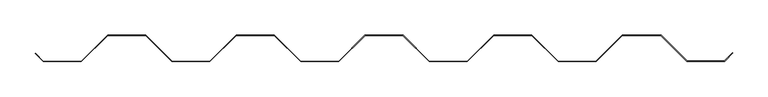
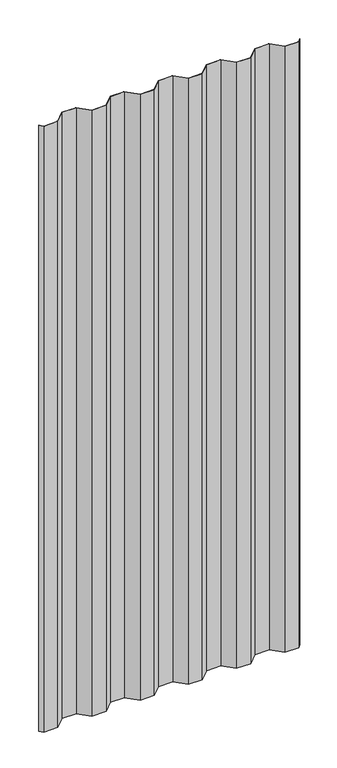
"""IFC4 building model written with IfcOpenShell, lengths in millimetres: proxy geometry, MBCI 7.2-V Panel-1 : MBCI 7.2-V Panel-1."""

import ifcopenshell
import ifcopenshell.guid

model = None  # the IFC model being written
_history = None  # IfcOwnerHistory: only IFC2X3 demands one
_inside = {}  # id of a spatial element -> (the spatial element, [elements in it])
_under = {}  # id of a project, library or spatial element -> (it, [spatial elements below it])
_declared = {}  # id of a project -> (the project, [libraries it declares])
_typed = {}  # id of a type object -> (the type object, [elements of that type])
_made_of = {}  # id of a material, layer set ... -> (it, [elements and type objects made of it])


def new_model(schema):
    """Start an empty IFC model of exactly this schema.

    Asked for "IFC4X3", IfcOpenShell would pick the latest addendum, in which some entities
    have other attributes; the version numbers below select the first issue.
    IFC2X3 requires an IfcOwnerHistory on every rooted entity: one is made here for all.
    """
    global model, _history
    if schema == "IFC4X3":
        model = ifcopenshell.file(schema_version=(4, 3, 0, 0))
    else:
        model = ifcopenshell.file(schema=schema)
    _inside.clear()
    _under.clear()
    _declared.clear()
    _typed.clear()
    _made_of.clear()
    _history = None
    if model.schema == "IFC2X3":
        org = make("IfcOrganization", Name="unknown")
        user = make(
            "IfcPersonAndOrganization",
            ThePerson=make("IfcPerson", FamilyName="unknown"),
            TheOrganization=org,
        )
        app = make(
            "IfcApplication",
            ApplicationDeveloper=org,
            Version="unknown",
            ApplicationFullName="unknown",
            ApplicationIdentifier="unknown",
        )
        _history = make(
            "IfcOwnerHistory",
            OwningUser=user,
            OwningApplication=app,
            ChangeAction="ADDED",
            CreationDate=0,
        )
    return model


def make(cls, **values):
    """One entity of the class cls with the attributes given. An attribute that is None is left unset."""
    return model.create_entity(
        cls, **{name: value for name, value in values.items() if value is not None}
    )


def rooted(cls, **values):
    """An entity with a GlobalId (a new one), such as an element, a storey or a relation."""
    return make(cls, GlobalId=ifcopenshell.guid.new(), OwnerHistory=_history, **values)


def si_unit(unit_type, name, prefix=None):
    """IfcSIUnit, for example si_unit("LENGTHUNIT", "METRE", prefix="MILLI")."""
    return make("IfcSIUnit", UnitType=unit_type, Prefix=prefix, Name=name)


def assignment(units):
    """IfcUnitAssignment: the units of a project."""
    return None if units is None else make("IfcUnitAssignment", Units=units)


def point(xyz):
    """IfcCartesianPoint."""
    return None if xyz is None else make("IfcCartesianPoint", Coordinates=xyz)


def direction(xyz):
    """IfcDirection."""
    return None if xyz is None else make("IfcDirection", DirectionRatios=xyz)


def frame(location, z_axis=None, x_axis=None):
    """IfcAxis2Placement3D, a coordinate frame: its origin and axes. An axis left out is left unset."""
    return make(
        "IfcAxis2Placement3D",
        Location=point(location),
        Axis=direction(z_axis),
        RefDirection=direction(x_axis),
    )


def origin():
    """The frame at (0, 0, 0) with its axes left unset."""
    return frame((0.0, 0.0, 0.0))


def place(relative_to, where):
    """IfcLocalPlacement: puts the frame where relative to a parent placement (None: the world)."""
    return make(
        "IfcLocalPlacement", PlacementRelTo=relative_to, RelativePlacement=where
    )


def context(
    kind, dimensions, precision=None, world=None, true_north=None, identifier=None
):
    """IfcGeometricRepresentationContext, for example the 3D "Model" context."""
    return make(
        "IfcGeometricRepresentationContext",
        ContextIdentifier=identifier,
        ContextType=kind,
        CoordinateSpaceDimension=dimensions,
        Precision=precision,
        WorldCoordinateSystem=world,
        TrueNorth=true_north,
    )


def project(units=None, contexts=None):
    """IfcProject with its units and contexts."""
    return rooted(
        "IfcProject",
        Name="project",
        RepresentationContexts=contexts,
        UnitsInContext=assignment(units),
    )


def spatial(cls, under=None, at=None, **own):
    """A site, building, storey or space (cls), placed at a placement, below another one or the project."""
    s = rooted(cls, ObjectPlacement=at, **own)
    if under is not None:
        _under.setdefault(under.id(), (under, []))[1].append(s)
    return s


def polyline(points):
    """IfcPolyline through the points."""
    return make("IfcPolyline", Points=[point(p) for p in points])


def outline(outer, holes=None, kind="AREA"):
    """IfcArbitraryClosedProfileDef: a profile drawn as a closed curve; with holes, ...WithVoids."""
    if holes is None:
        return make("IfcArbitraryClosedProfileDef", ProfileType=kind, OuterCurve=outer)
    return make(
        "IfcArbitraryProfileDefWithVoids",
        ProfileType=kind,
        OuterCurve=outer,
        InnerCurves=holes,
    )


def extrude(swept, where, along, depth):
    """IfcExtrudedAreaSolid: the profile swept, set in the frame where, extruded along a direction by depth."""
    return make(
        "IfcExtrudedAreaSolid",
        SweptArea=swept,
        Position=where,
        ExtrudedDirection=direction(along),
        Depth=depth,
    )


def shape(context_of_items, identifier, shape_type, items):
    """IfcShapeRepresentation: the items that make up one representation, for example the "Body"."""
    return make(
        "IfcShapeRepresentation",
        ContextOfItems=context_of_items,
        RepresentationIdentifier=identifier,
        RepresentationType=shape_type,
        Items=items,
    )


def source(mapping_origin, context_of_items, identifier, shape_type, items):
    """IfcRepresentationMap: a shape defined once, which mapped items show again and again."""
    return make(
        "IfcRepresentationMap",
        MappingOrigin=mapping_origin,
        MappedRepresentation=shape(context_of_items, identifier, shape_type, items),
    )


def transform(
    local_origin,
    x_axis=None,
    y_axis=None,
    z_axis=None,
    scale=None,
    scale2=None,
    scale3=None,
    uniform=True,
):
    """IfcCartesianTransformationOperator3D, or its non-uniform kind. x_axis, y_axis, z_axis: its Axis1, 2, 3."""
    if uniform:
        return make(
            "IfcCartesianTransformationOperator3D",
            Axis1=direction(x_axis),
            Axis2=direction(y_axis),
            LocalOrigin=point(local_origin),
            Scale=scale,
            Axis3=direction(z_axis),
        )
    return make(
        "IfcCartesianTransformationOperator3DnonUniform",
        Axis1=direction(x_axis),
        Axis2=direction(y_axis),
        LocalOrigin=point(local_origin),
        Scale=scale,
        Axis3=direction(z_axis),
        Scale2=scale2,
        Scale3=scale3,
    )


def mapped(mapping_source, mapping_target):
    """IfcMappedItem: shows the shape of a source again, moved by a transform."""
    return make(
        "IfcMappedItem", MappingSource=mapping_source, MappingTarget=mapping_target
    )


def made_of(thing, what):
    """Note that an element or type object is made of a material, layer set ...; save() writes the relation."""
    if what is not None:
        _made_of.setdefault(what.id(), (what, []))[1].append(thing)
    return thing


def element(
    cls,
    number,
    at=None,
    inside=None,
    cuts=None,
    type_object=None,
    material=None,
    context=None,
    identifier="Body",
    shape_type=None,
    held_by="IfcProductDefinitionShape",
    body=None,
    shapes=None,
    **own,
):
    """One element of the class cls, such as IfcWall. Its Tag is "e" and its number.

    at: its placement. inside: the storey or other place that contains it. cuts: it is an
    opening in that element (IfcRelVoidsElement). A single representation is given by context,
    identifier, shape_type and body (its items); several are given by shapes. held_by: the class
    of the entity that holds the representations. save() writes the other relations.
    """
    e = rooted(cls, Tag="e%d" % number, ObjectPlacement=at, **own)
    if body is not None:
        shapes = [shape(context, identifier, shape_type, body)]
    if shapes is not None:
        e.Representation = make(held_by, Representations=shapes)
    if inside is not None:
        _inside.setdefault(inside.id(), (inside, []))[1].append(e)
    if cuts is not None:
        rooted(
            "IfcRelVoidsElement", RelatingBuildingElement=cuts, RelatedOpeningElement=e
        )
    if type_object is not None:
        _typed.setdefault(type_object.id(), (type_object, []))[1].append(e)
    return made_of(e, material)


def aggregate(whole, parts):
    """IfcRelAggregates: a whole, such as a stair, and the parts it consists of."""
    return rooted("IfcRelAggregates", RelatingObject=whole, RelatedObjects=parts)


def save(model, path):
    """Write the relations noted so far, then the file.

    IfcRelAggregates (storeys below a building ...), IfcRelContainedInSpatialStructure (elements
    in a storey), IfcRelDefinesByType, IfcRelAssociatesMaterial and IfcRelDeclares: one each for
    every whole, place, type object, material and project.
    """
    for whole, parts in _under.values():
        aggregate(whole, parts)
    for where, things in _inside.values():
        rooted(
            "IfcRelContainedInSpatialStructure",
            RelatedElements=things,
            RelatingStructure=where,
        )
    for kind, things in _typed.values():
        rooted("IfcRelDefinesByType", RelatedObjects=things, RelatingType=kind)
    for what, things in _made_of.values():
        rooted("IfcRelAssociatesMaterial", RelatedObjects=things, RelatingMaterial=what)
    for by, libraries in _declared.values():
        rooted("IfcRelDeclares", RelatingContext=by, RelatedDefinitions=libraries)
    model.write(path)


def generic_models_de5cb4ec(model_context):
    return source(origin(), model_context, "Body", "SweptSolid", [
        extrude(outline(polyline([(589155.5303729, -531639.2163841), (589101.4186638, -531639.2163841), (589090.0180296, -531627.81575), (589090.8180038, -531627.7738251), (589101.6652503, -531638.6210716), (589155.2837864, -531638.6210716), (589192.7741864, -531601.1306716), (589247.0548503, -531601.1306716), (589284.5452503, -531638.6210716), (589338.1637864, -531638.6210716), (589375.6541864, -531601.1306716), (589429.9348503, -531601.1306716), (589467.4252503, -531638.6210716), (589521.0437864, -531638.6210716), (589558.5341864, -531601.1306716), (589612.8148503, -531601.1306716), (589650.3052503, -531638.6210716), (589703.9237864, -531638.6210716), (589741.4141864, -531601.1306716), (589795.6948503, -531601.1306716), (589833.1852503, -531638.6210716), (589886.8037864, -531638.6210716), (589924.2941864, -531601.1306716), (589979.4384503, -531601.1306716), (590016.3192503, -531638.0114716), (590069.4073773, -531638.0114716), (590080.5378112, -531626.8810377), (590081.3246865, -531626.9360614), (590069.6539638, -531638.6067841), (590016.0726638, -531638.6067841), (589979.1918638, -531601.7259841), (589924.5407729, -531601.7259841), (589887.0503729, -531639.2163841), (589832.9386638, -531639.2163841), (589795.4482638, -531601.7259841), (589741.6607729, -531601.7259841), (589704.1703729, -531639.2163841), (589650.0586638, -531639.2163841), (589612.5682638, -531601.7259841), (589558.7807729, -531601.7259841), (589521.2903729, -531639.2163841), (589467.1786638, -531639.2163841), (589429.6882638, -531601.7259841), (589375.9007729, -531601.7259841), (589338.4103729, -531639.2163841), (589284.2986638, -531639.2163841), (589246.8082638, -531601.7259841), (589193.0207729, -531601.7259841), (589155.5303729, -531639.2163841)])), frame((0.0, 0.0, 6.35), z_axis=(0.0, 0.0, 1.0), x_axis=(1.0, 0.0, 0.0)), (0.0, 0.0, 1.0), 2432.05),
    ])


if __name__ == "__main__":
    model = new_model("IFC4")
    model_context = context("Model", 3, world=origin())
    ifc_project = project(units=[si_unit("LENGTHUNIT", "METRE", prefix="MILLI")], contexts=[model_context])
    site = spatial("IfcSite", under=ifc_project)
    building = spatial("IfcBuilding", under=site)
    placement = place(None, origin())
    generic_models_shape = generic_models_de5cb4ec(model_context)
    element("IfcBuildingElementProxy", 1, Name="MBCI 7.2-V Panel-1 : MBCI 7.2-V Panel-1", ObjectType="MBCI 7.2-V Panel-1 : MBCI 7.2-V Panel-1", at=placement, inside=building, context=model_context, shape_type="MappedRepresentation", body=[
        mapped(generic_models_shape, transform((0.0, 0.0, 0.0), x_axis=(1.0, 0.0, 0.0), y_axis=(0.0, 1.0, 0.0), z_axis=(0.0, 0.0, 1.0))),
    ])
    save(model, "model.ifc")

# Revit data of these elements
# Element 1 (IfcBuildingElementProxy, "MBCI 7.2-V Panel-1 : MBCI 7.2-V Panel-1")
#   Materials on its faces: "MTL PANEL"
# Materials
#   "MTL PANEL": class "Generic", colour RGB 239 242 240, transparency 0, Cost = 0
